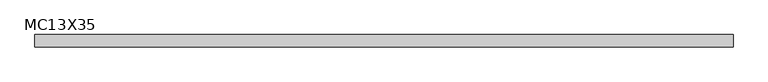
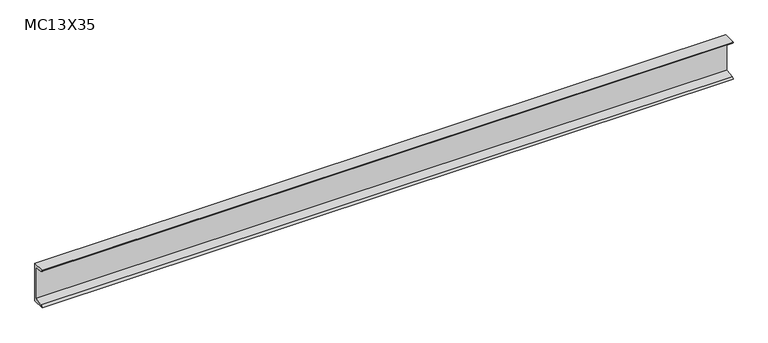
"""IFC4 building model written with IfcOpenShell, lengths in millimetres: beam geometry, MC-Miscellaneous Channel : MC13X35."""

import ifcopenshell
import ifcopenshell.guid

model = None  # the IFC model being written
_history = None  # IfcOwnerHistory: only IFC2X3 demands one
_inside = {}  # id of a spatial element -> (the spatial element, [elements in it])
_under = {}  # id of a project, library or spatial element -> (it, [spatial elements below it])
_declared = {}  # id of a project -> (the project, [libraries it declares])
_typed = {}  # id of a type object -> (the type object, [elements of that type])
_made_of = {}  # id of a material, layer set ... -> (it, [elements and type objects made of it])


def new_model(schema):
    """Start an empty IFC model of exactly this schema.

    Asked for "IFC4X3", IfcOpenShell would pick the latest addendum, in which some entities
    have other attributes; the version numbers below select the first issue.
    IFC2X3 requires an IfcOwnerHistory on every rooted entity: one is made here for all.
    """
    global model, _history
    if schema == "IFC4X3":
        model = ifcopenshell.file(schema_version=(4, 3, 0, 0))
    else:
        model = ifcopenshell.file(schema=schema)
    _inside.clear()
    _under.clear()
    _declared.clear()
    _typed.clear()
    _made_of.clear()
    _history = None
    if model.schema == "IFC2X3":
        org = make("IfcOrganization", Name="unknown")
        user = make(
            "IfcPersonAndOrganization",
            ThePerson=make("IfcPerson", FamilyName="unknown"),
            TheOrganization=org,
        )
        app = make(
            "IfcApplication",
            ApplicationDeveloper=org,
            Version="unknown",
            ApplicationFullName="unknown",
            ApplicationIdentifier="unknown",
        )
        _history = make(
            "IfcOwnerHistory",
            OwningUser=user,
            OwningApplication=app,
            ChangeAction="ADDED",
            CreationDate=0,
        )
    return model


def make(cls, **values):
    """One entity of the class cls with the attributes given. An attribute that is None is left unset."""
    return model.create_entity(
        cls, **{name: value for name, value in values.items() if value is not None}
    )


def rooted(cls, **values):
    """An entity with a GlobalId (a new one), such as an element, a storey or a relation."""
    return make(cls, GlobalId=ifcopenshell.guid.new(), OwnerHistory=_history, **values)


def si_unit(unit_type, name, prefix=None):
    """IfcSIUnit, for example si_unit("LENGTHUNIT", "METRE", prefix="MILLI")."""
    return make("IfcSIUnit", UnitType=unit_type, Prefix=prefix, Name=name)


def assignment(units):
    """IfcUnitAssignment: the units of a project."""
    return None if units is None else make("IfcUnitAssignment", Units=units)


def point(xyz):
    """IfcCartesianPoint."""
    return None if xyz is None else make("IfcCartesianPoint", Coordinates=xyz)


def direction(xyz):
    """IfcDirection."""
    return None if xyz is None else make("IfcDirection", DirectionRatios=xyz)


def frame(location, z_axis=None, x_axis=None):
    """IfcAxis2Placement3D, a coordinate frame: its origin and axes. An axis left out is left unset."""
    return make(
        "IfcAxis2Placement3D",
        Location=point(location),
        Axis=direction(z_axis),
        RefDirection=direction(x_axis),
    )


def frame_2d(location, x_axis=None):
    """IfcAxis2Placement2D, a coordinate frame in the plane: its origin and x axis."""
    return make(
        "IfcAxis2Placement2D", Location=point(location), RefDirection=direction(x_axis)
    )


def origin():
    """The frame at (0, 0, 0) with its axes left unset."""
    return frame((0.0, 0.0, 0.0))


def place(relative_to, where):
    """IfcLocalPlacement: puts the frame where relative to a parent placement (None: the world)."""
    return make(
        "IfcLocalPlacement", PlacementRelTo=relative_to, RelativePlacement=where
    )


def context(
    kind, dimensions, precision=None, world=None, true_north=None, identifier=None
):
    """IfcGeometricRepresentationContext, for example the 3D "Model" context."""
    return make(
        "IfcGeometricRepresentationContext",
        ContextIdentifier=identifier,
        ContextType=kind,
        CoordinateSpaceDimension=dimensions,
        Precision=precision,
        WorldCoordinateSystem=world,
        TrueNorth=true_north,
    )


def project(units=None, contexts=None):
    """IfcProject with its units and contexts."""
    return rooted(
        "IfcProject",
        Name="project",
        RepresentationContexts=contexts,
        UnitsInContext=assignment(units),
    )


def spatial(cls, under=None, at=None, **own):
    """A site, building, storey or space (cls), placed at a placement, below another one or the project."""
    s = rooted(cls, ObjectPlacement=at, **own)
    if under is not None:
        _under.setdefault(under.id(), (under, []))[1].append(s)
    return s


def polyline(points):
    """IfcPolyline through the points."""
    return make("IfcPolyline", Points=[point(p) for p in points])


def circle_curve(where, radius):
    """IfcCircle in the frame where."""
    return make("IfcCircle", Position=where, Radius=radius)


def trimmed(basis, trim1, trim2, sense, master):
    """IfcTrimmedCurve: the piece of a basis curve between two trims."""
    return make(
        "IfcTrimmedCurve",
        BasisCurve=basis,
        Trim1=trim1,
        Trim2=trim2,
        SenseAgreement=sense,
        MasterRepresentation=master,
    )


def segment(curve, same_sense, transition):
    """IfcCompositeCurveSegment."""
    return make(
        "IfcCompositeCurveSegment",
        Transition=transition,
        SameSense=same_sense,
        ParentCurve=curve,
    )


def composite_curve(segments, self_intersect=None):
    """IfcCompositeCurve: segments joined end to end."""
    return make("IfcCompositeCurve", Segments=segments, SelfIntersect=self_intersect)


def outline(outer, holes=None, kind="AREA"):
    """IfcArbitraryClosedProfileDef: a profile drawn as a closed curve; with holes, ...WithVoids."""
    if holes is None:
        return make("IfcArbitraryClosedProfileDef", ProfileType=kind, OuterCurve=outer)
    return make(
        "IfcArbitraryProfileDefWithVoids",
        ProfileType=kind,
        OuterCurve=outer,
        InnerCurves=holes,
    )


def extrude(swept, where, along, depth):
    """IfcExtrudedAreaSolid: the profile swept, set in the frame where, extruded along a direction by depth."""
    return make(
        "IfcExtrudedAreaSolid",
        SweptArea=swept,
        Position=where,
        ExtrudedDirection=direction(along),
        Depth=depth,
    )


def shape(context_of_items, identifier, shape_type, items):
    """IfcShapeRepresentation: the items that make up one representation, for example the "Body"."""
    return make(
        "IfcShapeRepresentation",
        ContextOfItems=context_of_items,
        RepresentationIdentifier=identifier,
        RepresentationType=shape_type,
        Items=items,
    )


def source(mapping_origin, context_of_items, identifier, shape_type, items):
    """IfcRepresentationMap: a shape defined once, which mapped items show again and again."""
    return make(
        "IfcRepresentationMap",
        MappingOrigin=mapping_origin,
        MappedRepresentation=shape(context_of_items, identifier, shape_type, items),
    )


def transform(
    local_origin,
    x_axis=None,
    y_axis=None,
    z_axis=None,
    scale=None,
    scale2=None,
    scale3=None,
    uniform=True,
):
    """IfcCartesianTransformationOperator3D, or its non-uniform kind. x_axis, y_axis, z_axis: its Axis1, 2, 3."""
    if uniform:
        return make(
            "IfcCartesianTransformationOperator3D",
            Axis1=direction(x_axis),
            Axis2=direction(y_axis),
            LocalOrigin=point(local_origin),
            Scale=scale,
            Axis3=direction(z_axis),
        )
    return make(
        "IfcCartesianTransformationOperator3DnonUniform",
        Axis1=direction(x_axis),
        Axis2=direction(y_axis),
        LocalOrigin=point(local_origin),
        Scale=scale,
        Axis3=direction(z_axis),
        Scale2=scale2,
        Scale3=scale3,
    )


def mapped(mapping_source, mapping_target):
    """IfcMappedItem: shows the shape of a source again, moved by a transform."""
    return make(
        "IfcMappedItem", MappingSource=mapping_source, MappingTarget=mapping_target
    )


def made_of(thing, what):
    """Note that an element or type object is made of a material, layer set ...; save() writes the relation."""
    if what is not None:
        _made_of.setdefault(what.id(), (what, []))[1].append(thing)
    return thing


def element(
    cls,
    number,
    at=None,
    inside=None,
    cuts=None,
    type_object=None,
    material=None,
    context=None,
    identifier="Body",
    shape_type=None,
    held_by="IfcProductDefinitionShape",
    body=None,
    shapes=None,
    **own,
):
    """One element of the class cls, such as IfcWall. Its Tag is "e" and its number.

    at: its placement. inside: the storey or other place that contains it. cuts: it is an
    opening in that element (IfcRelVoidsElement). A single representation is given by context,
    identifier, shape_type and body (its items); several are given by shapes. held_by: the class
    of the entity that holds the representations. save() writes the other relations.
    """
    e = rooted(cls, Tag="e%d" % number, ObjectPlacement=at, **own)
    if body is not None:
        shapes = [shape(context, identifier, shape_type, body)]
    if shapes is not None:
        e.Representation = make(held_by, Representations=shapes)
    if inside is not None:
        _inside.setdefault(inside.id(), (inside, []))[1].append(e)
    if cuts is not None:
        rooted(
            "IfcRelVoidsElement", RelatingBuildingElement=cuts, RelatedOpeningElement=e
        )
    if type_object is not None:
        _typed.setdefault(type_object.id(), (type_object, []))[1].append(e)
    return made_of(e, material)


def aggregate(whole, parts):
    """IfcRelAggregates: a whole, such as a stair, and the parts it consists of."""
    return rooted("IfcRelAggregates", RelatingObject=whole, RelatedObjects=parts)


def save(model, path):
    """Write the relations noted so far, then the file.

    IfcRelAggregates (storeys below a building ...), IfcRelContainedInSpatialStructure (elements
    in a storey), IfcRelDefinesByType, IfcRelAssociatesMaterial and IfcRelDeclares: one each for
    every whole, place, type object, material and project.
    """
    for whole, parts in _under.values():
        aggregate(whole, parts)
    for where, things in _inside.values():
        rooted(
            "IfcRelContainedInSpatialStructure",
            RelatedElements=things,
            RelatingStructure=where,
        )
    for kind, things in _typed.values():
        rooted("IfcRelDefinesByType", RelatedObjects=things, RelatingType=kind)
    for what, things in _made_of.values():
        rooted("IfcRelAssociatesMaterial", RelatedObjects=things, RelatingMaterial=what)
    for by, libraries in _declared.values():
        rooted("IfcRelDeclares", RelatingContext=by, RelatedDefinitions=libraries)
    model.write(path)


def mc13x35_caec82c8(model_context):
    return source(origin(), model_context, "Body", "SweptSolid", [
        extrude(outline(composite_curve([segment(polyline([(24.892, 165.1), (24.892, -165.1), (-78.486, -165.1)]), True, "CONTINUOUS"), segment(trimmed(circle_curve(frame_2d((-62.992, -165.1)), 15.494), [point((-78.486, -165.1))], [point((-62.992, -149.606))], False, "CARTESIAN"), True, "CONTINUOUS"), segment(polyline([(-62.992, -149.606), (13.5382, -137.4848071), (13.5382, 137.4848071), (-62.992, 149.606)]), True, "CONTINUOUS"), segment(trimmed(circle_curve(frame_2d((-62.992, 165.1)), 15.494), [point((-62.992, 149.606))], [point((-78.486, 165.1))], False, "CARTESIAN"), True, "CONTINUOUS"), segment(polyline([(-78.486, 165.1), (24.892, 165.1)]), True, "CONTINUOUS")], self_intersect=False)), frame((-2728.468, 0.0, 0.0), z_axis=(1.0, 0.0, 0.0), x_axis=(0.0, 1.0, 0.0)), (0.0, 0.0, 1.0), 5763.768),
    ])


if __name__ == "__main__":
    model = new_model("IFC4")
    model_context = context("Model", 3, world=origin())
    ifc_project = project(units=[si_unit("LENGTHUNIT", "METRE", prefix="MILLI")], contexts=[model_context])
    site = spatial("IfcSite", under=ifc_project)
    building = spatial("IfcBuilding", under=site)
    placement = place(None, origin())
    mc13x35_shape = mc13x35_caec82c8(model_context)
    element("IfcBeam", 1, ObjectType="MC-Miscellaneous Channel : MC13X35", at=placement, inside=building, context=model_context, shape_type="MappedRepresentation", body=[
        mapped(mc13x35_shape, transform((0.0, 0.0, 0.0), x_axis=(1.0, 0.0, 0.0), y_axis=(0.0, 1.0, 0.0), z_axis=(0.0, 0.0, 1.0))),
    ])
    save(model, "model.ifc")

# Revit data of these elements
# Type "MC-Miscellaneous Channel : MC13X35"
#   Assembly Code = "B10"
#   W = 35
#   Length [instance default] = 5' - 0"
#   bf = 0' - 4.07"
#   d = 1' - 1"
#   tf = 0' - 0.61"
#   tw = 0' - 0.447"
#   x = 0' - 0.98"
#   A = 0.0715278 SF
#   Structural Material [instance default] = Steel ASTM A36
# Element 1 (IfcBeam, "MC-Miscellaneous Channel : MC13X35")
#   Structural Material = Steel ASTM A992
#   Materials on its faces: "Steel ASTM A992"
# Materials
#   "Steel ASTM A36": class "Metal", colour RGB 199 199 199, transparency 0, Description = "Structural steel, ASTM A36 Grade B, mill finish", Cost = 0
#   "Steel ASTM A992": class "Metal", colour RGB 199 199 199, transparency 0, Description = "Structural steel 50ksi", Cost = 0
